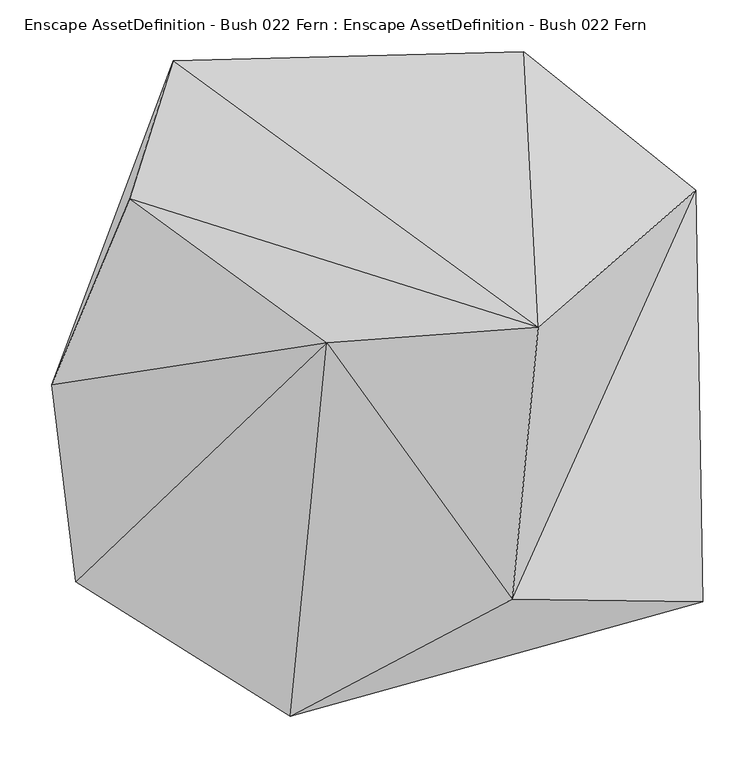
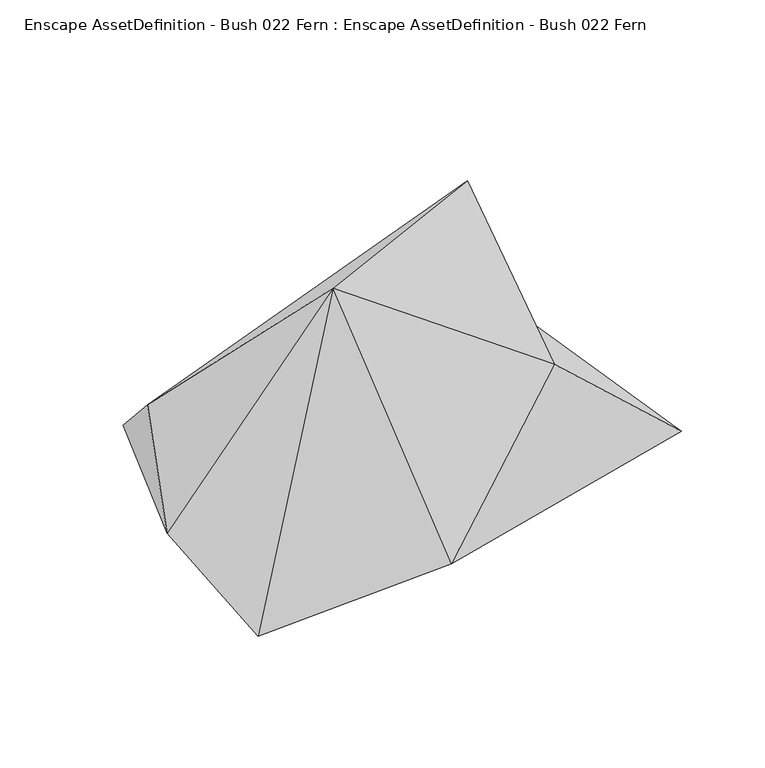
"""IFC4 building model written with IfcOpenShell, lengths in millimetres: geographic element geometry, Enscape AssetDefinition - Bush 022 Fern : Enscape AssetDefinition - Bush 022 Fern."""

import ifcopenshell
import ifcopenshell.guid

model = None  # the IFC model being written
_history = None  # IfcOwnerHistory: only IFC2X3 demands one
_inside = {}  # id of a spatial element -> (the spatial element, [elements in it])
_under = {}  # id of a project, library or spatial element -> (it, [spatial elements below it])
_declared = {}  # id of a project -> (the project, [libraries it declares])
_typed = {}  # id of a type object -> (the type object, [elements of that type])
_made_of = {}  # id of a material, layer set ... -> (it, [elements and type objects made of it])


def new_model(schema):
    """Start an empty IFC model of exactly this schema.

    Asked for "IFC4X3", IfcOpenShell would pick the latest addendum, in which some entities
    have other attributes; the version numbers below select the first issue.
    IFC2X3 requires an IfcOwnerHistory on every rooted entity: one is made here for all.
    """
    global model, _history
    if schema == "IFC4X3":
        model = ifcopenshell.file(schema_version=(4, 3, 0, 0))
    else:
        model = ifcopenshell.file(schema=schema)
    _inside.clear()
    _under.clear()
    _declared.clear()
    _typed.clear()
    _made_of.clear()
    _history = None
    if model.schema == "IFC2X3":
        org = make("IfcOrganization", Name="unknown")
        user = make(
            "IfcPersonAndOrganization",
            ThePerson=make("IfcPerson", FamilyName="unknown"),
            TheOrganization=org,
        )
        app = make(
            "IfcApplication",
            ApplicationDeveloper=org,
            Version="unknown",
            ApplicationFullName="unknown",
            ApplicationIdentifier="unknown",
        )
        _history = make(
            "IfcOwnerHistory",
            OwningUser=user,
            OwningApplication=app,
            ChangeAction="ADDED",
            CreationDate=0,
        )
    return model


def make(cls, **values):
    """One entity of the class cls with the attributes given. An attribute that is None is left unset."""
    return model.create_entity(
        cls, **{name: value for name, value in values.items() if value is not None}
    )


def rooted(cls, **values):
    """An entity with a GlobalId (a new one), such as an element, a storey or a relation."""
    return make(cls, GlobalId=ifcopenshell.guid.new(), OwnerHistory=_history, **values)


def si_unit(unit_type, name, prefix=None):
    """IfcSIUnit, for example si_unit("LENGTHUNIT", "METRE", prefix="MILLI")."""
    return make("IfcSIUnit", UnitType=unit_type, Prefix=prefix, Name=name)


def assignment(units):
    """IfcUnitAssignment: the units of a project."""
    return None if units is None else make("IfcUnitAssignment", Units=units)


def point(xyz):
    """IfcCartesianPoint."""
    return None if xyz is None else make("IfcCartesianPoint", Coordinates=xyz)


def direction(xyz):
    """IfcDirection."""
    return None if xyz is None else make("IfcDirection", DirectionRatios=xyz)


def frame(location, z_axis=None, x_axis=None):
    """IfcAxis2Placement3D, a coordinate frame: its origin and axes. An axis left out is left unset."""
    return make(
        "IfcAxis2Placement3D",
        Location=point(location),
        Axis=direction(z_axis),
        RefDirection=direction(x_axis),
    )


def origin():
    """The frame at (0, 0, 0) with its axes left unset."""
    return frame((0.0, 0.0, 0.0))


def place(relative_to, where):
    """IfcLocalPlacement: puts the frame where relative to a parent placement (None: the world)."""
    return make(
        "IfcLocalPlacement", PlacementRelTo=relative_to, RelativePlacement=where
    )


def context(
    kind, dimensions, precision=None, world=None, true_north=None, identifier=None
):
    """IfcGeometricRepresentationContext, for example the 3D "Model" context."""
    return make(
        "IfcGeometricRepresentationContext",
        ContextIdentifier=identifier,
        ContextType=kind,
        CoordinateSpaceDimension=dimensions,
        Precision=precision,
        WorldCoordinateSystem=world,
        TrueNorth=true_north,
    )


def project(units=None, contexts=None):
    """IfcProject with its units and contexts."""
    return rooted(
        "IfcProject",
        Name="project",
        RepresentationContexts=contexts,
        UnitsInContext=assignment(units),
    )


def spatial(cls, under=None, at=None, **own):
    """A site, building, storey or space (cls), placed at a placement, below another one or the project."""
    s = rooted(cls, ObjectPlacement=at, **own)
    if under is not None:
        _under.setdefault(under.id(), (under, []))[1].append(s)
    return s


def faces_of(points, faces, orient=None, outer=None):
    """IfcFace entities. A face is a list of loops; a loop is a list of indices into points, from 0.

    orient and outer hold one flag for each loop. By default every Orientation is true, the
    first loop of a face is its IfcFaceOuterBound and the others are IfcFaceBound.
    """
    made = []
    for i, loops in enumerate(faces):
        bounds = []
        for j, loop in enumerate(loops):
            is_outer = j == 0 if outer is None else outer[i][j]
            bounds.append(
                make(
                    "IfcFaceOuterBound" if is_outer else "IfcFaceBound",
                    Bound=make("IfcPolyLoop", Polygon=[points[k] for k in loop]),
                    Orientation=True if orient is None else orient[i][j],
                )
            )
        made.append(make("IfcFace", Bounds=bounds))
    return made


def faceted_brep(points, faces, orient=None, outer=None, voids=None):
    """IfcFacetedBrep: a solid bounded by flat faces; with voids (closed shells), ...WithVoids."""
    shared = [point(p) for p in points]
    hull = make("IfcClosedShell", CfsFaces=faces_of(shared, faces, orient, outer))
    if voids is None:
        return make("IfcFacetedBrep", Outer=hull)
    return make(
        "IfcFacetedBrepWithVoids",
        Outer=hull,
        Voids=[
            make(cls, CfsFaces=faces_of(shared, fs, o, b)) for cls, fs, o, b in voids
        ],
    )


def shape(context_of_items, identifier, shape_type, items):
    """IfcShapeRepresentation: the items that make up one representation, for example the "Body"."""
    return make(
        "IfcShapeRepresentation",
        ContextOfItems=context_of_items,
        RepresentationIdentifier=identifier,
        RepresentationType=shape_type,
        Items=items,
    )


def source(mapping_origin, context_of_items, identifier, shape_type, items):
    """IfcRepresentationMap: a shape defined once, which mapped items show again and again."""
    return make(
        "IfcRepresentationMap",
        MappingOrigin=mapping_origin,
        MappedRepresentation=shape(context_of_items, identifier, shape_type, items),
    )


def transform(
    local_origin,
    x_axis=None,
    y_axis=None,
    z_axis=None,
    scale=None,
    scale2=None,
    scale3=None,
    uniform=True,
):
    """IfcCartesianTransformationOperator3D, or its non-uniform kind. x_axis, y_axis, z_axis: its Axis1, 2, 3."""
    if uniform:
        return make(
            "IfcCartesianTransformationOperator3D",
            Axis1=direction(x_axis),
            Axis2=direction(y_axis),
            LocalOrigin=point(local_origin),
            Scale=scale,
            Axis3=direction(z_axis),
        )
    return make(
        "IfcCartesianTransformationOperator3DnonUniform",
        Axis1=direction(x_axis),
        Axis2=direction(y_axis),
        LocalOrigin=point(local_origin),
        Scale=scale,
        Axis3=direction(z_axis),
        Scale2=scale2,
        Scale3=scale3,
    )


def mapped(mapping_source, mapping_target):
    """IfcMappedItem: shows the shape of a source again, moved by a transform."""
    return make(
        "IfcMappedItem", MappingSource=mapping_source, MappingTarget=mapping_target
    )


def made_of(thing, what):
    """Note that an element or type object is made of a material, layer set ...; save() writes the relation."""
    if what is not None:
        _made_of.setdefault(what.id(), (what, []))[1].append(thing)
    return thing


def element(
    cls,
    number,
    at=None,
    inside=None,
    cuts=None,
    type_object=None,
    material=None,
    context=None,
    identifier="Body",
    shape_type=None,
    held_by="IfcProductDefinitionShape",
    body=None,
    shapes=None,
    **own,
):
    """One element of the class cls, such as IfcWall. Its Tag is "e" and its number.

    at: its placement. inside: the storey or other place that contains it. cuts: it is an
    opening in that element (IfcRelVoidsElement). A single representation is given by context,
    identifier, shape_type and body (its items); several are given by shapes. held_by: the class
    of the entity that holds the representations. save() writes the other relations.
    """
    e = rooted(cls, Tag="e%d" % number, ObjectPlacement=at, **own)
    if body is not None:
        shapes = [shape(context, identifier, shape_type, body)]
    if shapes is not None:
        e.Representation = make(held_by, Representations=shapes)
    if inside is not None:
        _inside.setdefault(inside.id(), (inside, []))[1].append(e)
    if cuts is not None:
        rooted(
            "IfcRelVoidsElement", RelatingBuildingElement=cuts, RelatedOpeningElement=e
        )
    if type_object is not None:
        _typed.setdefault(type_object.id(), (type_object, []))[1].append(e)
    return made_of(e, material)


def aggregate(whole, parts):
    """IfcRelAggregates: a whole, such as a stair, and the parts it consists of."""
    return rooted("IfcRelAggregates", RelatingObject=whole, RelatedObjects=parts)


def save(model, path):
    """Write the relations noted so far, then the file.

    IfcRelAggregates (storeys below a building ...), IfcRelContainedInSpatialStructure (elements
    in a storey), IfcRelDefinesByType, IfcRelAssociatesMaterial and IfcRelDeclares: one each for
    every whole, place, type object, material and project.
    """
    for whole, parts in _under.values():
        aggregate(whole, parts)
    for where, things in _inside.values():
        rooted(
            "IfcRelContainedInSpatialStructure",
            RelatedElements=things,
            RelatingStructure=where,
        )
    for kind, things in _typed.values():
        rooted("IfcRelDefinesByType", RelatedObjects=things, RelatingType=kind)
    for what, things in _made_of.values():
        rooted("IfcRelAssociatesMaterial", RelatedObjects=things, RelatingMaterial=what)
    for by, libraries in _declared.values():
        rooted("IfcRelDeclares", RelatingContext=by, RelatedDefinitions=libraries)
    model.write(path)


def enscape_assetdefinition_bush_022_fern_enscape_16470abe(model_context):
    return source(origin(), model_context, "Body", "Brep", [
        faceted_brep([(-237.1029854, 165.6155586, 164.089337), (-47.436472, 26.9630011, 361.0720038), (156.4911604, 41.8980867, 446.0159242), (-312.0678067, -13.4198414, 101.9497737), (-289.0363634, -203.1974643, 50.9199388), (131.4267814, -220.2729434, 331.5717876), (-82.5495422, -332.7048719, 168.5667038), (142.4339563, 306.9921732, 28.7053473), (308.2143664, 173.6044735, 108.4637195), (0.0, 0.0, -3.9840727), (314.9578571, -222.6221114, 165.6070352), (-195.3037977, 298.6308336, 37.6759209)], [[[0, 1, 2]], [[3, 1, 0]], [[4, 1, 3]], [[5, 1, 6]], [[2, 1, 5]], [[7, 2, 8]], [[4, 3, 9]], [[8, 5, 10]], [[2, 7, 11]], [[4, 10, 6]], [[5, 8, 2]], [[10, 9, 8]], [[8, 9, 7]], [[4, 9, 10]], [[9, 3, 11]], [[9, 11, 7]], [[6, 10, 5]], [[6, 1, 4]], [[3, 0, 11]], [[0, 2, 11]]]),
    ])


if __name__ == "__main__":
    model = new_model("IFC4")
    model_context = context("Model", 3, world=origin())
    ifc_project = project(units=[si_unit("LENGTHUNIT", "METRE", prefix="MILLI")], contexts=[model_context])
    site = spatial("IfcSite", under=ifc_project)
    building = spatial("IfcBuilding", under=site)
    placement = place(None, origin())
    enscape_assetdefinition_bush_022_fern_enscape_shape = enscape_assetdefinition_bush_022_fern_enscape_16470abe(model_context)
    element("IfcGeographicElement", 1, ObjectType="Enscape AssetDefinition - Bush 022 Fern : Enscape AssetDefinition - Bush 022 Fern", at=placement, inside=building, context=model_context, shape_type="MappedRepresentation", body=[
        mapped(enscape_assetdefinition_bush_022_fern_enscape_shape, transform((0.0, 0.0, 0.0), x_axis=(1.0, 0.0, 0.0), y_axis=(0.0, 1.0, 0.0), z_axis=(0.0, 0.0, 1.0))),
    ])
    save(model, "model.ifc")

# Revit data of these elements
# Project information
#   Project Issue Date = "Issue Date"
#   Project Status = "Project Status"
#   Client Name = "Owner"
#   Project Address = "Enter address here"
#   Project Name = "Project Name"
#   Project Number = "0001"
# Type "Enscape AssetDefinition - Bush 022 Fern : Enscape AssetDefinition - Bush 022 Fern"
#   EnscapeAssetSource = "REMOTE"
#   EnscapeAssetId = "ca3fb51f-7cfd-4e9f-8287-cedadb532316"
#   Height = 0.446016 m
#   EnscapeNativeAssetHeight = 0.446016 m
#   Default Elevation = 0
